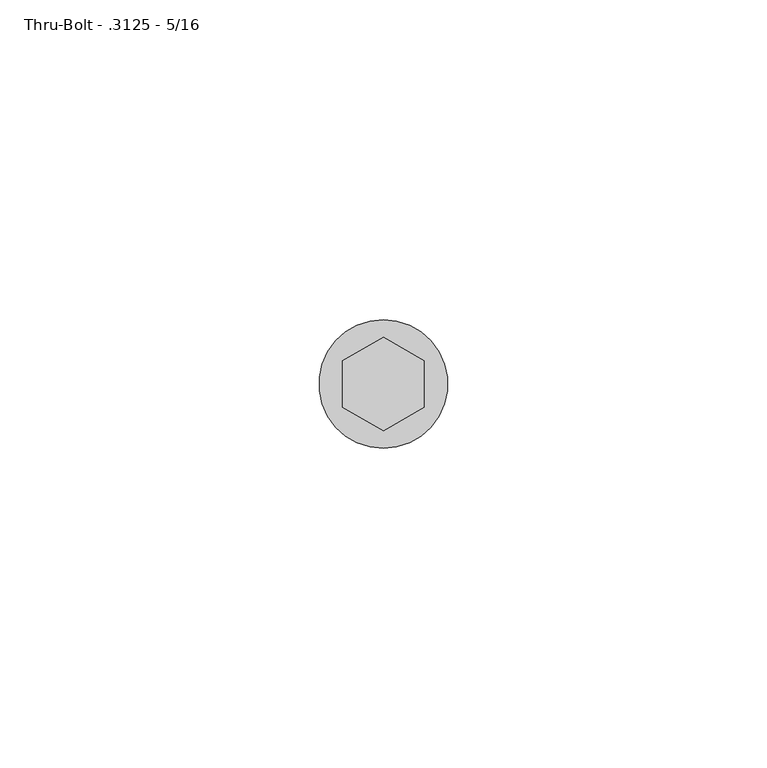
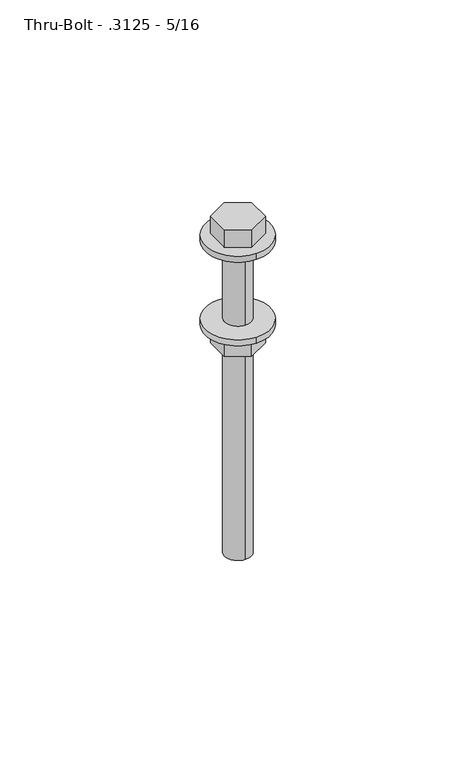
"""IFC4 building model written with IfcOpenShell, lengths in millimetres: fastener geometry, 060523 - W_P_C - Fastenings - Generic : Thru-Bolt - .3125 - 5/16."""

import ifcopenshell
import ifcopenshell.guid

model = None  # the IFC model being written
_history = None  # IfcOwnerHistory: only IFC2X3 demands one
_inside = {}  # id of a spatial element -> (the spatial element, [elements in it])
_under = {}  # id of a project, library or spatial element -> (it, [spatial elements below it])
_declared = {}  # id of a project -> (the project, [libraries it declares])
_typed = {}  # id of a type object -> (the type object, [elements of that type])
_made_of = {}  # id of a material, layer set ... -> (it, [elements and type objects made of it])


def new_model(schema):
    """Start an empty IFC model of exactly this schema.

    Asked for "IFC4X3", IfcOpenShell would pick the latest addendum, in which some entities
    have other attributes; the version numbers below select the first issue.
    IFC2X3 requires an IfcOwnerHistory on every rooted entity: one is made here for all.
    """
    global model, _history
    if schema == "IFC4X3":
        model = ifcopenshell.file(schema_version=(4, 3, 0, 0))
    else:
        model = ifcopenshell.file(schema=schema)
    _inside.clear()
    _under.clear()
    _declared.clear()
    _typed.clear()
    _made_of.clear()
    _history = None
    if model.schema == "IFC2X3":
        org = make("IfcOrganization", Name="unknown")
        user = make(
            "IfcPersonAndOrganization",
            ThePerson=make("IfcPerson", FamilyName="unknown"),
            TheOrganization=org,
        )
        app = make(
            "IfcApplication",
            ApplicationDeveloper=org,
            Version="unknown",
            ApplicationFullName="unknown",
            ApplicationIdentifier="unknown",
        )
        _history = make(
            "IfcOwnerHistory",
            OwningUser=user,
            OwningApplication=app,
            ChangeAction="ADDED",
            CreationDate=0,
        )
    return model


def make(cls, **values):
    """One entity of the class cls with the attributes given. An attribute that is None is left unset."""
    return model.create_entity(
        cls, **{name: value for name, value in values.items() if value is not None}
    )


def rooted(cls, **values):
    """An entity with a GlobalId (a new one), such as an element, a storey or a relation."""
    return make(cls, GlobalId=ifcopenshell.guid.new(), OwnerHistory=_history, **values)


def si_unit(unit_type, name, prefix=None):
    """IfcSIUnit, for example si_unit("LENGTHUNIT", "METRE", prefix="MILLI")."""
    return make("IfcSIUnit", UnitType=unit_type, Prefix=prefix, Name=name)


def assignment(units):
    """IfcUnitAssignment: the units of a project."""
    return None if units is None else make("IfcUnitAssignment", Units=units)


def point(xyz):
    """IfcCartesianPoint."""
    return None if xyz is None else make("IfcCartesianPoint", Coordinates=xyz)


def direction(xyz):
    """IfcDirection."""
    return None if xyz is None else make("IfcDirection", DirectionRatios=xyz)


def frame(location, z_axis=None, x_axis=None):
    """IfcAxis2Placement3D, a coordinate frame: its origin and axes. An axis left out is left unset."""
    return make(
        "IfcAxis2Placement3D",
        Location=point(location),
        Axis=direction(z_axis),
        RefDirection=direction(x_axis),
    )


def frame_2d(location, x_axis=None):
    """IfcAxis2Placement2D, a coordinate frame in the plane: its origin and x axis."""
    return make(
        "IfcAxis2Placement2D", Location=point(location), RefDirection=direction(x_axis)
    )


def origin():
    """The frame at (0, 0, 0) with its axes left unset."""
    return frame((0.0, 0.0, 0.0))


def origin_with_axes():
    """The frame at (0, 0, 0) with the z axis (0, 0, 1) and the x axis (1, 0, 0) written out."""
    return frame((0.0, 0.0, 0.0), z_axis=(0.0, 0.0, 1.0), x_axis=(1.0, 0.0, 0.0))


def origin_2d():
    """The frame at (0, 0) in the plane with its x axis left unset."""
    return frame_2d((0.0, 0.0))


def place(relative_to, where):
    """IfcLocalPlacement: puts the frame where relative to a parent placement (None: the world)."""
    return make(
        "IfcLocalPlacement", PlacementRelTo=relative_to, RelativePlacement=where
    )


def context(
    kind, dimensions, precision=None, world=None, true_north=None, identifier=None
):
    """IfcGeometricRepresentationContext, for example the 3D "Model" context."""
    return make(
        "IfcGeometricRepresentationContext",
        ContextIdentifier=identifier,
        ContextType=kind,
        CoordinateSpaceDimension=dimensions,
        Precision=precision,
        WorldCoordinateSystem=world,
        TrueNorth=true_north,
    )


def project(units=None, contexts=None):
    """IfcProject with its units and contexts."""
    return rooted(
        "IfcProject",
        Name="project",
        RepresentationContexts=contexts,
        UnitsInContext=assignment(units),
    )


def spatial(cls, under=None, at=None, **own):
    """A site, building, storey or space (cls), placed at a placement, below another one or the project."""
    s = rooted(cls, ObjectPlacement=at, **own)
    if under is not None:
        _under.setdefault(under.id(), (under, []))[1].append(s)
    return s


def polyline(points):
    """IfcPolyline through the points."""
    return make("IfcPolyline", Points=[point(p) for p in points])


def circle_curve(where, radius):
    """IfcCircle in the frame where."""
    return make("IfcCircle", Position=where, Radius=radius)


def trimmed(basis, trim1, trim2, sense, master):
    """IfcTrimmedCurve: the piece of a basis curve between two trims."""
    return make(
        "IfcTrimmedCurve",
        BasisCurve=basis,
        Trim1=trim1,
        Trim2=trim2,
        SenseAgreement=sense,
        MasterRepresentation=master,
    )


def segment(curve, same_sense, transition):
    """IfcCompositeCurveSegment."""
    return make(
        "IfcCompositeCurveSegment",
        Transition=transition,
        SameSense=same_sense,
        ParentCurve=curve,
    )


def composite_curve(segments, self_intersect=None):
    """IfcCompositeCurve: segments joined end to end."""
    return make("IfcCompositeCurve", Segments=segments, SelfIntersect=self_intersect)


def outline(outer, holes=None, kind="AREA"):
    """IfcArbitraryClosedProfileDef: a profile drawn as a closed curve; with holes, ...WithVoids."""
    if holes is None:
        return make("IfcArbitraryClosedProfileDef", ProfileType=kind, OuterCurve=outer)
    return make(
        "IfcArbitraryProfileDefWithVoids",
        ProfileType=kind,
        OuterCurve=outer,
        InnerCurves=holes,
    )


def extrude(swept, where, along, depth):
    """IfcExtrudedAreaSolid: the profile swept, set in the frame where, extruded along a direction by depth."""
    return make(
        "IfcExtrudedAreaSolid",
        SweptArea=swept,
        Position=where,
        ExtrudedDirection=direction(along),
        Depth=depth,
    )


def shape(context_of_items, identifier, shape_type, items):
    """IfcShapeRepresentation: the items that make up one representation, for example the "Body"."""
    return make(
        "IfcShapeRepresentation",
        ContextOfItems=context_of_items,
        RepresentationIdentifier=identifier,
        RepresentationType=shape_type,
        Items=items,
    )


def source(mapping_origin, context_of_items, identifier, shape_type, items):
    """IfcRepresentationMap: a shape defined once, which mapped items show again and again."""
    return make(
        "IfcRepresentationMap",
        MappingOrigin=mapping_origin,
        MappedRepresentation=shape(context_of_items, identifier, shape_type, items),
    )


def transform(
    local_origin,
    x_axis=None,
    y_axis=None,
    z_axis=None,
    scale=None,
    scale2=None,
    scale3=None,
    uniform=True,
):
    """IfcCartesianTransformationOperator3D, or its non-uniform kind. x_axis, y_axis, z_axis: its Axis1, 2, 3."""
    if uniform:
        return make(
            "IfcCartesianTransformationOperator3D",
            Axis1=direction(x_axis),
            Axis2=direction(y_axis),
            LocalOrigin=point(local_origin),
            Scale=scale,
            Axis3=direction(z_axis),
        )
    return make(
        "IfcCartesianTransformationOperator3DnonUniform",
        Axis1=direction(x_axis),
        Axis2=direction(y_axis),
        LocalOrigin=point(local_origin),
        Scale=scale,
        Axis3=direction(z_axis),
        Scale2=scale2,
        Scale3=scale3,
    )


def mapped(mapping_source, mapping_target):
    """IfcMappedItem: shows the shape of a source again, moved by a transform."""
    return make(
        "IfcMappedItem", MappingSource=mapping_source, MappingTarget=mapping_target
    )


def made_of(thing, what):
    """Note that an element or type object is made of a material, layer set ...; save() writes the relation."""
    if what is not None:
        _made_of.setdefault(what.id(), (what, []))[1].append(thing)
    return thing


def element(
    cls,
    number,
    at=None,
    inside=None,
    cuts=None,
    type_object=None,
    material=None,
    context=None,
    identifier="Body",
    shape_type=None,
    held_by="IfcProductDefinitionShape",
    body=None,
    shapes=None,
    **own,
):
    """One element of the class cls, such as IfcWall. Its Tag is "e" and its number.

    at: its placement. inside: the storey or other place that contains it. cuts: it is an
    opening in that element (IfcRelVoidsElement). A single representation is given by context,
    identifier, shape_type and body (its items); several are given by shapes. held_by: the class
    of the entity that holds the representations. save() writes the other relations.
    """
    e = rooted(cls, Tag="e%d" % number, ObjectPlacement=at, **own)
    if body is not None:
        shapes = [shape(context, identifier, shape_type, body)]
    if shapes is not None:
        e.Representation = make(held_by, Representations=shapes)
    if inside is not None:
        _inside.setdefault(inside.id(), (inside, []))[1].append(e)
    if cuts is not None:
        rooted(
            "IfcRelVoidsElement", RelatingBuildingElement=cuts, RelatedOpeningElement=e
        )
    if type_object is not None:
        _typed.setdefault(type_object.id(), (type_object, []))[1].append(e)
    return made_of(e, material)


def aggregate(whole, parts):
    """IfcRelAggregates: a whole, such as a stair, and the parts it consists of."""
    return rooted("IfcRelAggregates", RelatingObject=whole, RelatedObjects=parts)


def save(model, path):
    """Write the relations noted so far, then the file.

    IfcRelAggregates (storeys below a building ...), IfcRelContainedInSpatialStructure (elements
    in a storey), IfcRelDefinesByType, IfcRelAssociatesMaterial and IfcRelDeclares: one each for
    every whole, place, type object, material and project.
    """
    for whole, parts in _under.values():
        aggregate(whole, parts)
    for where, things in _inside.values():
        rooted(
            "IfcRelContainedInSpatialStructure",
            RelatedElements=things,
            RelatingStructure=where,
        )
    for kind, things in _typed.values():
        rooted("IfcRelDefinesByType", RelatedObjects=things, RelatingType=kind)
    for what, things in _made_of.values():
        rooted("IfcRelAssociatesMaterial", RelatedObjects=things, RelatingMaterial=what)
    for by, libraries in _declared.values():
        rooted("IfcRelDeclares", RelatingContext=by, RelatedDefinitions=libraries)
    model.write(path)


def thru_bolt_3125_5_16_4cf2d9be(model_context):
    return source(origin(), model_context, "Body", "SweptSolid", [
        extrude(outline(composite_curve([segment(trimmed(circle_curve(origin_2d(), 10.067925), [point((0.0, 10.067925))], [point((0.0, -10.067925))], False, "CARTESIAN"), True, "CONTINUOUS"), segment(trimmed(circle_curve(origin_2d(), 10.067925), [point((0.0, -10.067925))], [point((0.0, 10.067925))], False, "CARTESIAN"), True, "CONTINUOUS")], self_intersect=False)), origin_with_axes(), (0.0, 0.0, 1.0), 1.984375),
        extrude(outline(composite_curve([segment(trimmed(circle_curve(origin_2d(), 10.067925), [point((0.0, 10.067925))], [point((0.0, -10.067925))], False, "CARTESIAN"), True, "CONTINUOUS"), segment(trimmed(circle_curve(origin_2d(), 10.067925), [point((0.0, -10.067925))], [point((0.0, 10.067925))], False, "CARTESIAN"), True, "CONTINUOUS")], self_intersect=False)), frame((0.0, 0.0, -27.384375), z_axis=(0.0, 0.0, 1.0), x_axis=(1.0, 0.0, 0.0)), (0.0, 0.0, 1.0), 1.984375),
        extrude(outline(polyline([(-6.35, -3.6661742), (-6.35, 3.6661742), (0.0, 7.3323484), (6.35, 3.6661742), (6.35, -3.6661742), (0.0, -7.3323484), (-6.35, -3.6661742)])), frame((0.0, 0.0, -33.3375), z_axis=(0.0, 0.0, 1.0), x_axis=(1.0, 0.0, 0.0)), (0.0, 0.0, 1.0), 5.953125),
        extrude(outline(polyline([(-6.35, 3.6661742), (0.0, 7.3323484), (6.35, 3.6661742), (6.35, -3.6661742), (0.0, -7.3323484), (-6.35, -3.6661742), (-6.35, 3.6661742)])), frame((0.0, 0.0, 1.984375), z_axis=(0.0, 0.0, 1.0), x_axis=(1.0, 0.0, 0.0)), (0.0, 0.0, 1.0), 5.953125),
        extrude(outline(composite_curve([segment(trimmed(circle_curve(origin_2d(), 4.1148), [point((0.0, -4.1148))], [point((0.0, 4.1148))], False, "CARTESIAN"), True, "CONTINUOUS"), segment(trimmed(circle_curve(origin_2d(), 4.1148), [point((0.0, 4.1148))], [point((0.0, -4.1148))], False, "CARTESIAN"), True, "CONTINUOUS")], self_intersect=False)), frame((0.0, 0.0, -101.6), z_axis=(0.0, 0.0, 1.0), x_axis=(1.0, 0.0, 0.0)), (0.0, 0.0, 1.0), 103.584375),
    ])


if __name__ == "__main__":
    model = new_model("IFC4")
    model_context = context("Model", 3, world=origin())
    ifc_project = project(units=[si_unit("LENGTHUNIT", "METRE", prefix="MILLI")], contexts=[model_context])
    site = spatial("IfcSite", under=ifc_project)
    building = spatial("IfcBuilding", under=site)
    placement = place(None, origin())
    thru_bolt_3125_5_16_shape = thru_bolt_3125_5_16_4cf2d9be(model_context)
    element("IfcFastener", 1, ObjectType="060523 - W_P_C - Fastenings - Generic : Thru-Bolt - .3125 - 5/16", at=placement, inside=building, context=model_context, shape_type="MappedRepresentation", body=[
        mapped(thru_bolt_3125_5_16_shape, transform((0.0, 0.0, 0.0), x_axis=(1.0, 0.0, 0.0), y_axis=(0.0, 1.0, 0.0), z_axis=(0.0, 0.0, 1.0))),
    ])
    save(model, "model.ifc")

# Revit data of these elements
# Type "060523 - W_P_C - Fastenings - Generic : Thru-Bolt - .3125 - 5/16"
#   Washer_Thickness = 0' - 0 5/64"
#   Washer Radius = 0' - 0.39638"
#   Washer Offset - Head = 0' - 0 5/64"
#   Washer Offset = 0' - 0 5/64"
#   Thickness_of_Substrate [instance default] = 0' - 1"
#   Side = 0' - 0 37/128"
#   Radius = 0' - 0.162"
#   Length [instance default] = 0' - 4"
#   Head Size = 0' - 0 1/2"
#   Head Radius = 0' - 0 1/4"
#   Head Height = 0' - 0 15/64"
#   Double Diameter = 0' - 0.648"
#   Diameter = 0' - 0.324"
#   Default Elevation = 4' - 0"
#   Washer_Nut_Visibility = yes
#   Washer_Head_Visibility = yes
#   Round_Head_Visibility = no
#   Point Visibility = no
#   Nut_Visibility = yes
#   Hex_Head_Visiblilty = yes
#   Washer Material = none
#   Bolt Material (Size) = AT SILL - FASTENER AT 24" O.C.
# Element 1 (IfcFastener, "060523 - W_P_C - Fastenings - Generic : Thru-Bolt - .3125 - 5/16")
#   Materials on its faces: "AT SILL - FASTENER AT 24\" O.C."
# Materials
#   "AT SILL - FASTENER AT 24\" O.C.": class "Generic", colour RGB 120 120 120, transparency 0, Cost = 0
